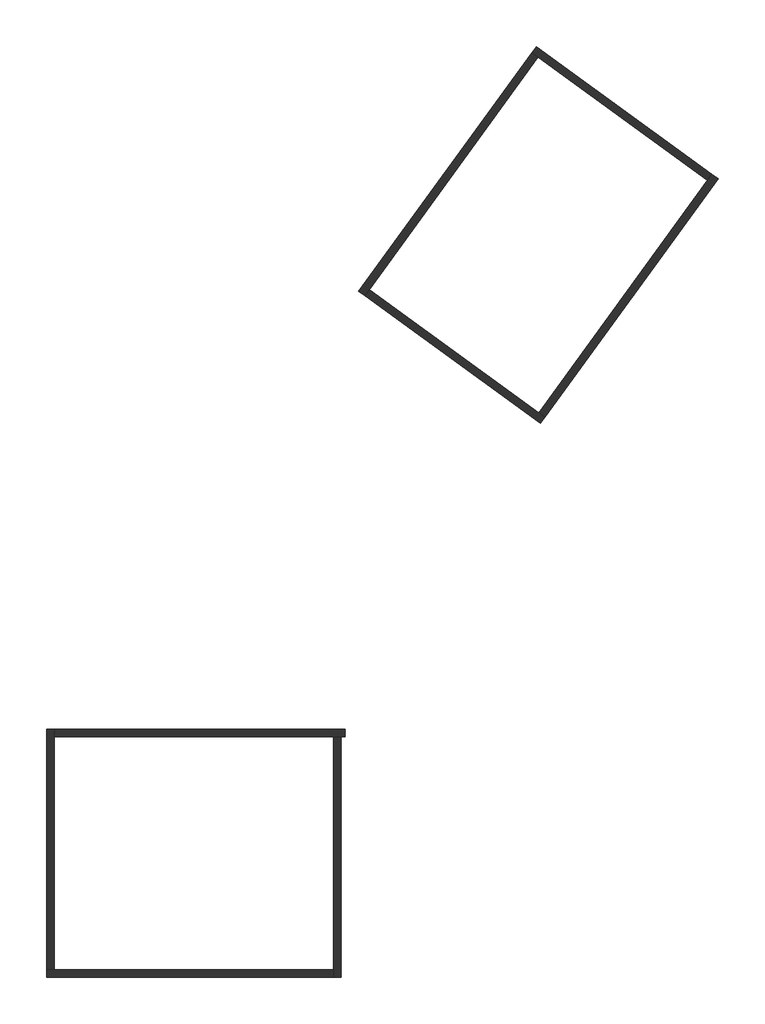
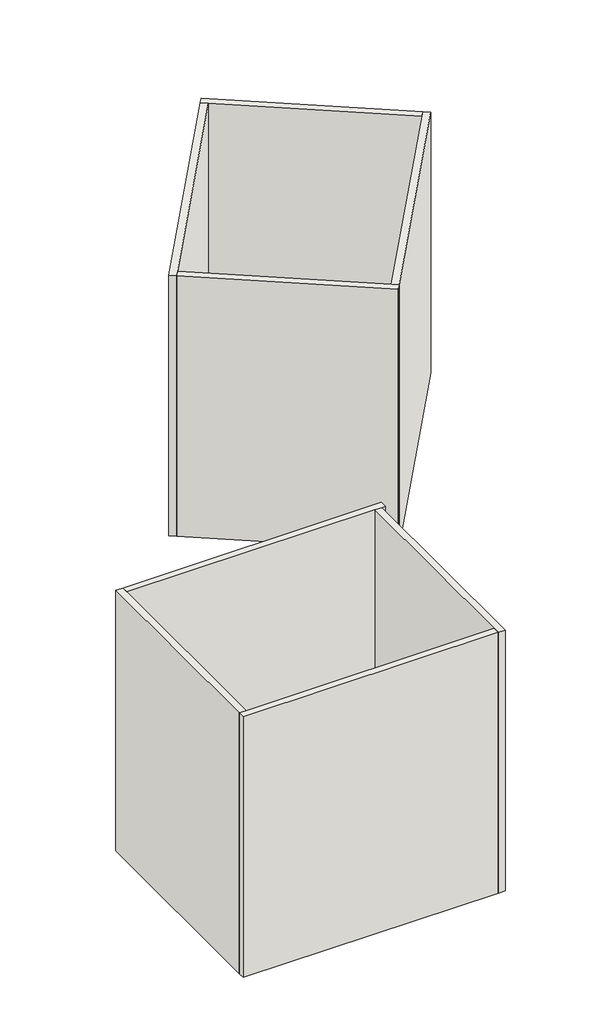
# One storey: 8 walls.
"""IFC4 building model written with IfcOpenShell, lengths in millimetres."""

import ifcopenshell
import ifcopenshell.guid

model = None  # the IFC model being written
_history = None  # IfcOwnerHistory: only IFC2X3 demands one
_inside = {}  # id of a spatial element -> (the spatial element, [elements in it])
_under = {}  # id of a project, library or spatial element -> (it, [spatial elements below it])
_declared = {}  # id of a project -> (the project, [libraries it declares])
_typed = {}  # id of a type object -> (the type object, [elements of that type])
_made_of = {}  # id of a material, layer set ... -> (it, [elements and type objects made of it])


def new_model(schema):
    """Start an empty IFC model of exactly this schema.

    Asked for "IFC4X3", IfcOpenShell would pick the latest addendum, in which some entities
    have other attributes; the version numbers below select the first issue.
    IFC2X3 requires an IfcOwnerHistory on every rooted entity: one is made here for all.
    """
    global model, _history
    if schema == "IFC4X3":
        model = ifcopenshell.file(schema_version=(4, 3, 0, 0))
    else:
        model = ifcopenshell.file(schema=schema)
    _inside.clear()
    _under.clear()
    _declared.clear()
    _typed.clear()
    _made_of.clear()
    _history = None
    if model.schema == "IFC2X3":
        org = make("IfcOrganization", Name="unknown")
        user = make(
            "IfcPersonAndOrganization",
            ThePerson=make("IfcPerson", FamilyName="unknown"),
            TheOrganization=org,
        )
        app = make(
            "IfcApplication",
            ApplicationDeveloper=org,
            Version="unknown",
            ApplicationFullName="unknown",
            ApplicationIdentifier="unknown",
        )
        _history = make(
            "IfcOwnerHistory",
            OwningUser=user,
            OwningApplication=app,
            ChangeAction="ADDED",
            CreationDate=0,
        )
    return model


def make(cls, **values):
    """One entity of the class cls with the attributes given. An attribute that is None is left unset."""
    return model.create_entity(
        cls, **{name: value for name, value in values.items() if value is not None}
    )


def rooted(cls, **values):
    """An entity with a GlobalId (a new one), such as an element, a storey or a relation."""
    return make(cls, GlobalId=ifcopenshell.guid.new(), OwnerHistory=_history, **values)


def si_unit(unit_type, name, prefix=None):
    """IfcSIUnit, for example si_unit("LENGTHUNIT", "METRE", prefix="MILLI")."""
    return make("IfcSIUnit", UnitType=unit_type, Prefix=prefix, Name=name)


def assignment(units):
    """IfcUnitAssignment: the units of a project."""
    return None if units is None else make("IfcUnitAssignment", Units=units)


def point(xyz):
    """IfcCartesianPoint."""
    return None if xyz is None else make("IfcCartesianPoint", Coordinates=xyz)


def direction(xyz):
    """IfcDirection."""
    return None if xyz is None else make("IfcDirection", DirectionRatios=xyz)


def frame(location, z_axis=None, x_axis=None):
    """IfcAxis2Placement3D, a coordinate frame: its origin and axes. An axis left out is left unset."""
    return make(
        "IfcAxis2Placement3D",
        Location=point(location),
        Axis=direction(z_axis),
        RefDirection=direction(x_axis),
    )


def origin():
    """The frame at (0, 0, 0) with its axes left unset."""
    return frame((0.0, 0.0, 0.0))


def place(relative_to, where):
    """IfcLocalPlacement: puts the frame where relative to a parent placement (None: the world)."""
    return make(
        "IfcLocalPlacement", PlacementRelTo=relative_to, RelativePlacement=where
    )


def context(
    kind, dimensions, precision=None, world=None, true_north=None, identifier=None
):
    """IfcGeometricRepresentationContext, for example the 3D "Model" context."""
    return make(
        "IfcGeometricRepresentationContext",
        ContextIdentifier=identifier,
        ContextType=kind,
        CoordinateSpaceDimension=dimensions,
        Precision=precision,
        WorldCoordinateSystem=world,
        TrueNorth=true_north,
    )


def project(units=None, contexts=None):
    """IfcProject with its units and contexts."""
    return rooted(
        "IfcProject",
        Name="project",
        RepresentationContexts=contexts,
        UnitsInContext=assignment(units),
    )


def spatial(cls, under=None, at=None, **own):
    """A site, building, storey or space (cls), placed at a placement, below another one or the project."""
    s = rooted(cls, ObjectPlacement=at, **own)
    if under is not None:
        _under.setdefault(under.id(), (under, []))[1].append(s)
    return s


def faces_of(points, faces, orient=None, outer=None):
    """IfcFace entities. A face is a list of loops; a loop is a list of indices into points, from 0.

    orient and outer hold one flag for each loop. By default every Orientation is true, the
    first loop of a face is its IfcFaceOuterBound and the others are IfcFaceBound.
    """
    made = []
    for i, loops in enumerate(faces):
        bounds = []
        for j, loop in enumerate(loops):
            is_outer = j == 0 if outer is None else outer[i][j]
            bounds.append(
                make(
                    "IfcFaceOuterBound" if is_outer else "IfcFaceBound",
                    Bound=make("IfcPolyLoop", Polygon=[points[k] for k in loop]),
                    Orientation=True if orient is None else orient[i][j],
                )
            )
        made.append(make("IfcFace", Bounds=bounds))
    return made


def faceted_brep(points, faces, orient=None, outer=None, voids=None):
    """IfcFacetedBrep: a solid bounded by flat faces; with voids (closed shells), ...WithVoids."""
    shared = [point(p) for p in points]
    hull = make("IfcClosedShell", CfsFaces=faces_of(shared, faces, orient, outer))
    if voids is None:
        return make("IfcFacetedBrep", Outer=hull)
    return make(
        "IfcFacetedBrepWithVoids",
        Outer=hull,
        Voids=[
            make(cls, CfsFaces=faces_of(shared, fs, o, b)) for cls, fs, o, b in voids
        ],
    )


def shape(context_of_items, identifier, shape_type, items):
    """IfcShapeRepresentation: the items that make up one representation, for example the "Body"."""
    return make(
        "IfcShapeRepresentation",
        ContextOfItems=context_of_items,
        RepresentationIdentifier=identifier,
        RepresentationType=shape_type,
        Items=items,
    )


def made_of(thing, what):
    """Note that an element or type object is made of a material, layer set ...; save() writes the relation."""
    if what is not None:
        _made_of.setdefault(what.id(), (what, []))[1].append(thing)
    return thing


def element(
    cls,
    number,
    at=None,
    inside=None,
    cuts=None,
    type_object=None,
    material=None,
    context=None,
    identifier="Body",
    shape_type=None,
    held_by="IfcProductDefinitionShape",
    body=None,
    shapes=None,
    **own,
):
    """One element of the class cls, such as IfcWall. Its Tag is "e" and its number.

    at: its placement. inside: the storey or other place that contains it. cuts: it is an
    opening in that element (IfcRelVoidsElement). A single representation is given by context,
    identifier, shape_type and body (its items); several are given by shapes. held_by: the class
    of the entity that holds the representations. save() writes the other relations.
    """
    e = rooted(cls, Tag="e%d" % number, ObjectPlacement=at, **own)
    if body is not None:
        shapes = [shape(context, identifier, shape_type, body)]
    if shapes is not None:
        e.Representation = make(held_by, Representations=shapes)
    if inside is not None:
        _inside.setdefault(inside.id(), (inside, []))[1].append(e)
    if cuts is not None:
        rooted(
            "IfcRelVoidsElement", RelatingBuildingElement=cuts, RelatedOpeningElement=e
        )
    if type_object is not None:
        _typed.setdefault(type_object.id(), (type_object, []))[1].append(e)
    return made_of(e, material)


def aggregate(whole, parts):
    """IfcRelAggregates: a whole, such as a stair, and the parts it consists of."""
    return rooted("IfcRelAggregates", RelatingObject=whole, RelatedObjects=parts)


def save(model, path):
    """Write the relations noted so far, then the file.

    IfcRelAggregates (storeys below a building ...), IfcRelContainedInSpatialStructure (elements
    in a storey), IfcRelDefinesByType, IfcRelAssociatesMaterial and IfcRelDeclares: one each for
    every whole, place, type object, material and project.
    """
    for whole, parts in _under.values():
        aggregate(whole, parts)
    for where, things in _inside.values():
        rooted(
            "IfcRelContainedInSpatialStructure",
            RelatedElements=things,
            RelatingStructure=where,
        )
    for kind, things in _typed.values():
        rooted("IfcRelDefinesByType", RelatedObjects=things, RelatingType=kind)
    for what, things in _made_of.values():
        rooted("IfcRelAssociatesMaterial", RelatedObjects=things, RelatingMaterial=what)
    for by, libraries in _declared.values():
        rooted("IfcRelDeclares", RelatingContext=by, RelatedDefinitions=libraries)
    model.write(path)


model = new_model("IFC4")

# Units and contexts
model_context = context("Model", 3, world=origin())
ifc_project = project(units=[si_unit("LENGTHUNIT", "METRE", prefix="MILLI")], contexts=[model_context])

# Site, building, storey
site = spatial("IfcSite", under=ifc_project)
building = spatial("IfcBuilding", under=site)
storey = spatial("IfcBuildingStorey", under=building, Name="Уровень 1", Elevation=0.0)

# Walls
placement = place(None, origin())
element("IfcWall", 1, ObjectType="Типовой - 200мм", at=placement, inside=storey, context=model_context, shape_type="Brep", body=[
    faceted_brep([(-4179.0520783, 10365.6524318, 0.0), (-4061.4950278, 10527.4558307, 0.0), (288.1158391, 16514.1815891, 0.0), (288.1158391, 16514.1815891, 8000.0), (-4061.4950278, 10527.4558307, 8000.0), (-4179.0520783, 10365.6524318, 8000.0), (-4340.8554772, 10483.2094823, 0.0), (-4340.8554772, 10483.2094823, 8000.0), (126.3124403, 16631.7386395, 8000.0), (126.3124403, 16631.7386395, 0.0)], [[[0, 1, 2, 3, 4, 5]], [[6, 7, 8, 9]], [[2, 1, 0, 6, 9]], [[5, 4, 3, 8, 7]], [[0, 5, 7, 6]], [[3, 2, 9, 8]]]),
])
element("IfcWall", 2, ObjectType="Типовой - 200мм", at=placement, inside=storey, context=model_context, shape_type="Brep", body=[
    faceted_brep([(469.0001407, 7235.8584179, 0.0), (307.1967418, 7353.4154683, 0.0), (-4061.4950278, 10527.4558307, 0.0), (-4061.4950278, 10527.4558307, 8000.0), (307.1967418, 7353.4154683, 8000.0), (469.0001407, 7235.8584179, 8000.0), (351.4430902, 7074.055019, 0.0), (351.4430902, 7074.055019, 8000.0), (-4179.0520783, 10365.6524318, 8000.0), (-4179.0520783, 10365.6524318, 0.0)], [[[0, 1, 2, 3, 4, 5]], [[6, 7, 8, 9]], [[2, 1, 0, 6, 9]], [[5, 4, 3, 8, 7]], [[0, 5, 7, 6]], [[3, 2, 9, 8]]]),
])
element("IfcWall", 3, ObjectType="Типовой - 200мм", at=placement, inside=storey, context=model_context, shape_type="Brep", body=[
    faceted_brep([(4774.3646592, 13501.9446256, 0.0), (4656.8076088, 13340.1412267, 0.0), (307.1967418, 7353.4154683, 0.0), (307.1967418, 7353.4154683, 8000.0), (4656.8076088, 13340.1412267, 8000.0), (4774.3646592, 13501.9446256, 8000.0), (4936.1680581, 13384.3875751, 0.0), (4936.1680581, 13384.3875751, 8000.0), (469.0001407, 7235.8584179, 8000.0), (469.0001407, 7235.8584179, 0.0)], [[[0, 1, 2, 3, 4, 5]], [[6, 7, 8, 9]], [[2, 1, 0, 6, 9]], [[5, 4, 3, 8, 7]], [[0, 5, 7, 6]], [[3, 2, 9, 8]]]),
])
element("IfcWall", 4, ObjectType="Типовой - 200мм", at=placement, inside=storey, context=model_context, shape_type="Brep", body=[
    faceted_brep([(126.3124403, 16631.7386395, 0.0), (288.1158391, 16514.1815891, 0.0), (4656.8076088, 13340.1412267, 0.0), (4656.8076088, 13340.1412267, 8000.0), (288.1158391, 16514.1815891, 8000.0), (126.3124403, 16631.7386395, 8000.0), (243.8694907, 16793.5420384, 0.0), (243.8694907, 16793.5420384, 8000.0), (4774.3646592, 13501.9446256, 8000.0), (4774.3646592, 13501.9446256, 0.0)], [[[0, 1, 2, 3, 4, 5]], [[6, 7, 8, 9]], [[2, 1, 0, 6, 9]], [[5, 4, 3, 8, 7]], [[0, 5, 7, 6]], [[3, 2, 9, 8]]]),
])
element("IfcWall", 5, ObjectType="Типовой - 200мм", at=placement, inside=storey, context=model_context, shape_type="Brep", body=[
    faceted_brep([(-4696.1840877, -809.2967894, 0.0), (-12196.1840877, -809.2967894, 0.0), (-12196.1840877, -809.2967894, 8000.0), (-4696.1840877, -809.2967894, 8000.0), (-4696.1840877, -1009.2967894, 0.0), (-4696.1840877, -1009.2967894, 8000.0), (-4796.1840877, -1009.2967894, 8000.0), (-4996.1840877, -1009.2967894, 8000.0), (-12196.1840877, -1009.2967894, 8000.0), (-12196.1840877, -1009.2967894, 0.0), (-4996.1840877, -1009.2967894, 0.0), (-4796.1840877, -1009.2967894, 0.0)], [[[0, 1, 2, 3]], [[4, 5, 6, 7, 8, 9, 10, 11]], [[1, 0, 4, 11, 10, 9]], [[3, 2, 8, 7, 6, 5]], [[0, 3, 5, 4]], [[2, 1, 9, 8]]]),
])
element("IfcWall", 6, ObjectType="Типовой - 200мм", at=placement, inside=storey, context=model_context, shape_type="Brep", body=[
    faceted_brep([(-4796.1840877, -7209.2967894, 0.0), (-4796.1840877, -1009.2967894, 0.0), (-4796.1840877, -1009.2967894, 8000.0), (-4796.1840877, -7209.2967894, 8000.0), (-4996.1840877, -7209.2967894, 0.0), (-4996.1840877, -7209.2967894, 8000.0), (-4996.1840877, -7009.2967894, 8000.0), (-4996.1840877, -1009.2967894, 8000.0), (-4996.1840877, -1009.2967894, 0.0), (-4996.1840877, -7009.2967894, 0.0)], [[[0, 1, 2, 3]], [[4, 5, 6, 7, 8, 9]], [[1, 0, 4, 9, 8]], [[3, 2, 7, 6, 5]], [[0, 3, 5, 4]], [[2, 1, 8, 7]]]),
])
element("IfcWall", 7, ObjectType="Типовой - 200мм", at=placement, inside=storey, context=model_context, shape_type="Brep", body=[
    faceted_brep([(-12396.1840877, -7209.2967894, 0.0), (-4996.1840877, -7209.2967894, 0.0), (-4996.1840877, -7209.2967894, 8000.0), (-12396.1840877, -7209.2967894, 8000.0), (-12396.1840877, -7009.2967894, 0.0), (-12396.1840877, -7009.2967894, 8000.0), (-12196.1840877, -7009.2967894, 8000.0), (-4996.1840877, -7009.2967894, 8000.0), (-4996.1840877, -7009.2967894, 0.0), (-12196.1840877, -7009.2967894, 0.0)], [[[0, 1, 2, 3]], [[4, 5, 6, 7, 8, 9]], [[1, 0, 4, 9, 8]], [[3, 2, 7, 6, 5]], [[0, 3, 5, 4]], [[2, 1, 8, 7]]]),
])
element("IfcWall", 8, ObjectType="Типовой - 200мм", at=placement, inside=storey, context=model_context, shape_type="Brep", body=[
    faceted_brep([(-12396.1840877, -809.2967894, 0.0), (-12396.1840877, -7009.2967894, 0.0), (-12396.1840877, -7009.2967894, 8000.0), (-12396.1840877, -809.2967894, 8000.0), (-12196.1840877, -809.2967894, 0.0), (-12196.1840877, -809.2967894, 8000.0), (-12196.1840877, -1009.2967894, 8000.0), (-12196.1840877, -7009.2967894, 8000.0), (-12196.1840877, -7009.2967894, 0.0), (-12196.1840877, -1009.2967894, 0.0)], [[[0, 1, 2, 3]], [[4, 5, 6, 7, 8, 9]], [[1, 0, 4, 9, 8]], [[3, 2, 7, 6, 5]], [[0, 3, 5, 4]], [[2, 1, 8, 7]]]),
])

save(model, "model.ifc")

# Revit data of these elements
# Project information
#   Дата утверждения проекта = "Дата выпуска"
#   Статус проекта = "Статус проекта"
#   Заказчик = "Владелец"
#   Адрес проекта = "Укажите адрес"
#   Наименование проекта = "Наименование проекта"
#   Номер проекта = "0001"
# Type "Типовой - 200мм"
#   Type Mark = "марка 1"
#   Layers, outside or top first: 200 mm no material (function 1)
# Elements 1, 2, 3, 4, 5, 6, 7, 8 (IfcWall, "Типовой - 200мм")
#   Top Offset = 0 mm
#   Base Offset = 0 mm
#   Unconnected Height = 8000 mm
#   wall height = 8000 mm
#   Phase Created = Стадия 1
#   Base Constraint = Уровень 1
#   Materials on its faces: "Стена по умолчанию"
# Materials
#   "Стена по умолчанию": class "Разное", colour RGB 128 128 128, transparency 0, Cost = 0
